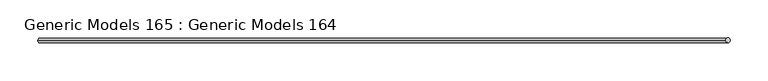
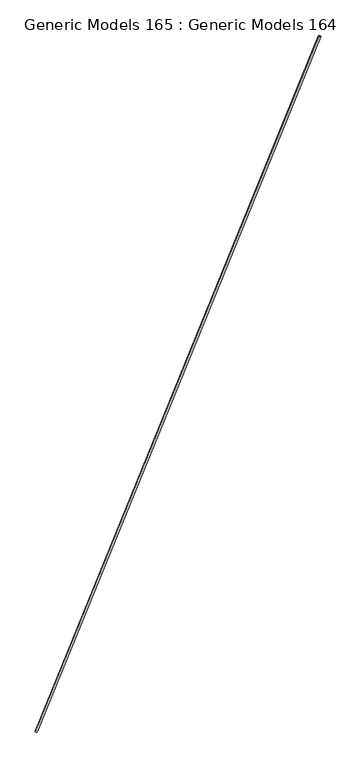
"""IFC4 building model written with IfcOpenShell, lengths in millimetres: proxy geometry, Generic Models 165 : Generic Models 164."""

from ifc_helpers import new_model, si_unit, point, frame, frame_2d, origin, place, context, project, spatial, circle_curve, trimmed, segment, composite_curve, outline, extrude, source, transform, mapped, element, save


def generic_models_165_generic_models_164_b4e33544(model_context):
    return source(origin(), model_context, "Body", "SweptSolid", [
        extrude(outline(composite_curve([segment(trimmed(circle_curve(frame_2d((0.0, -3.175)), 3.175), [point((0.0, -6.35))], [point((0.0, 0.0))], False, "CARTESIAN"), True, "CONTINUOUS"), segment(trimmed(circle_curve(frame_2d((0.0, -3.175)), 3.175), [point((0.0, 0.0))], [point((0.0, -6.35))], False, "CARTESIAN"), True, "CONTINUOUS")], self_intersect=False)), frame((33448.5989526, 41059.1932538, 266521.8196383), z_axis=(0.4071880938201211, 0.0, 0.9133443251321686), x_axis=(0.0, -1.0, 0.0)), (0.0, 0.0, 1.0), 2230.6570412),
    ])


if __name__ == "__main__":
    model = new_model("IFC4")
    model_context = context("Model", 3, world=origin())
    ifc_project = project(units=[si_unit("LENGTHUNIT", "METRE", prefix="MILLI")], contexts=[model_context])
    site = spatial("IfcSite", under=ifc_project)
    building = spatial("IfcBuilding", under=site)
    placement = place(None, origin())
    generic_models_165_generic_models_164_shape = generic_models_165_generic_models_164_b4e33544(model_context)
    element("IfcBuildingElementProxy", 1, Name="Generic Models 165 : Generic Models 164", ObjectType="Generic Models 165 : Generic Models 164", at=placement, inside=building, context=model_context, shape_type="MappedRepresentation", body=[
        mapped(generic_models_165_generic_models_164_shape, transform((0.0, 0.0, 0.0), x_axis=(1.0, 0.0, 0.0), y_axis=(0.0, 1.0, 0.0), z_axis=(0.0, 0.0, 1.0))),
    ])
    save(model, "model.ifc")

# Revit data of these elements
# Element 1 (IfcBuildingElementProxy, "Generic Models 165 : Generic Models 164")
#   Materials on its faces: "1/4\" GALV ROD - TURNBUCKLES - EYEHOOKS"
# Materials
#   "1/4\" GALV ROD - TURNBUCKLES - EYEHOOKS": class "Metal", colour RGB 199 199 199, transparency 0, Description = "Structural steel, ASTM A36 Grade B, mill finish", Cost = 0
